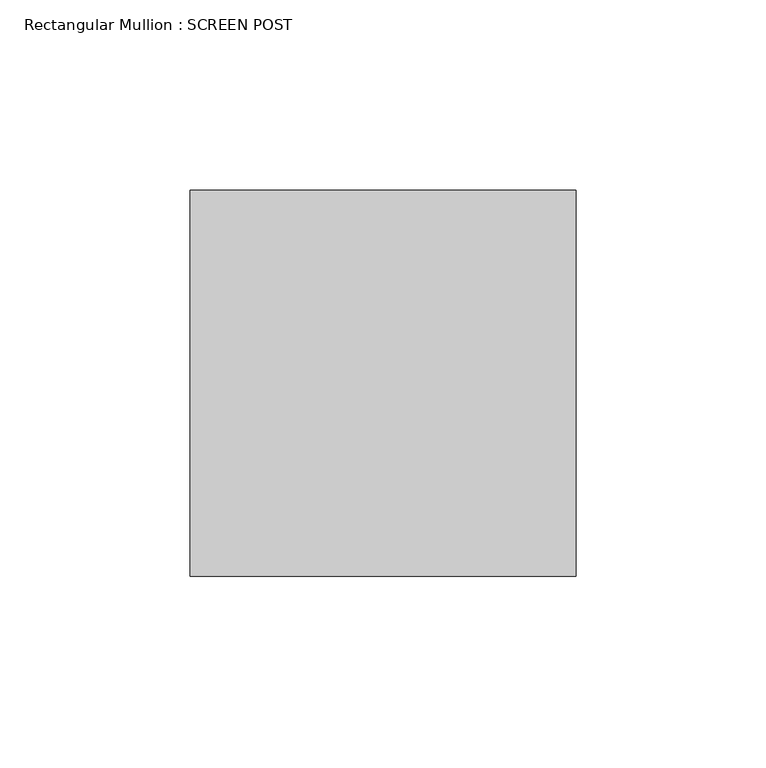
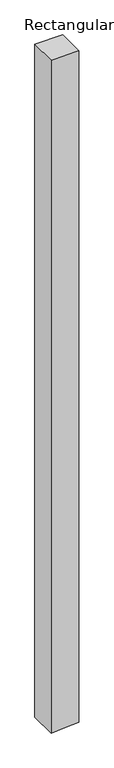
"""IFC4 building model written with IfcOpenShell, lengths in millimetres: member geometry, Rectangular Mullion : SCREEN POST."""

from ifc_helpers import new_model, si_unit, frame, origin, place, context, project, spatial, polyline, outline, extrude, source, transform, mapped, element, save


def rectangular_mullion_screen_post_0d75b437(model_context):
    return source(origin(), model_context, "Body", "SweptSolid", [
        extrude(outline(polyline([(0.0, 50.8), (0.0, -50.8), (-2585.9097052, -50.8), (-2583.126501, -6.3490391), (-2579.548233, 50.8), (0.0, 50.8)])), frame((0.0, -50.8, 0.0), z_axis=(0.0, 1.0, 0.0), x_axis=(0.0, 0.0, 1.0)), (0.0, 0.0, 1.0), 101.6),
    ])


if __name__ == "__main__":
    model = new_model("IFC4")
    model_context = context("Model", 3, world=origin())
    ifc_project = project(units=[si_unit("LENGTHUNIT", "METRE", prefix="MILLI")], contexts=[model_context])
    site = spatial("IfcSite", under=ifc_project)
    building = spatial("IfcBuilding", under=site)
    placement = place(None, origin())
    rectangular_mullion_screen_post_shape = rectangular_mullion_screen_post_0d75b437(model_context)
    element("IfcMember", 1, ObjectType="Rectangular Mullion : SCREEN POST", at=placement, inside=building, context=model_context, shape_type="MappedRepresentation", body=[
        mapped(rectangular_mullion_screen_post_shape, transform((0.0, 0.0, 0.0), x_axis=(1.0, 0.0, 0.0), y_axis=(0.0, 1.0, 0.0), z_axis=(0.0, 0.0, 1.0))),
    ])
    save(model, "model.ifc")

# Revit data of these elements
# Type "Rectangular Mullion : SCREEN POST"
#   built-in parameter 1007304 = 0.333333 (stored number, unit not read)
#   built-in parameter 1007301 = 0.166667 (stored number, unit not read)
#   built-in parameter 1007300 = 0.166667 (stored number, unit not read)
# Element 1 (IfcMember, "Rectangular Mullion : SCREEN POST")
#   Materials on its faces: "SCREEN PORCH FRAMING"
# Materials
#   "SCREEN PORCH FRAMING": class "Wood", colour RGB 164 134 123, transparency 0, Description = "Pinus Echinata", Cost = 0
